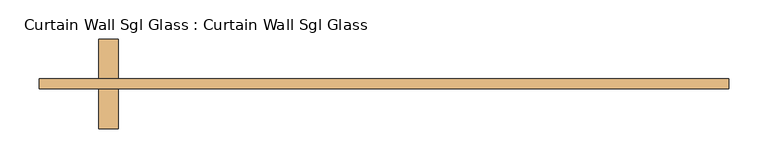
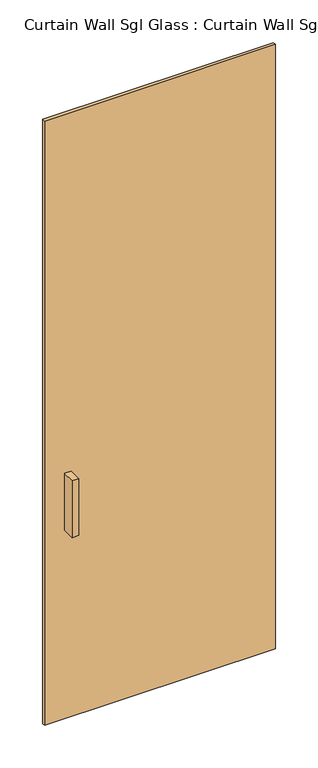
"""IFC4 building model written with IfcOpenShell, lengths in millimetres: door geometry, Curtain Wall Sgl Glass : Curtain Wall Sgl Glass."""

from ifc_helpers import new_model, si_unit, frame, origin, origin_with_axes, place, context, project, spatial, polyline, outline, extrude, source, transform, mapped, element, save


def curtain_wall_sgl_glass_curtain_wall_sgl_glass_0d6a1b13(model_context):
    return source(origin(), model_context, "Body", "SweptSolid", [
        extrude(outline(polyline([(-339.725, -12.7), (-365.125, -12.7), (-365.125, 38.1), (-339.725, 38.1), (-339.725, -12.7)])), frame((0.0, 0.0, 762.0), z_axis=(0.0, 0.0, 1.0), x_axis=(1.0, 0.0, 0.0)), (0.0, 0.0, 1.0), 228.6),
        extrude(outline(polyline([(-365.125, 101.6), (-339.725, 101.6), (-339.725, 50.8), (-365.125, 50.8), (-365.125, 101.6)])), frame((0.0, 0.0, 762.0), z_axis=(0.0, 0.0, 1.0), x_axis=(1.0, 0.0, 0.0)), (0.0, 0.0, 1.0), 228.6),
        extrude(outline(polyline([(441.325, 50.8), (441.325, 38.1), (-441.325, 38.1), (-441.325, 50.8), (441.325, 50.8)])), origin_with_axes(), (0.0, 0.0, 1.0), 2438.4),
    ])


if __name__ == "__main__":
    model = new_model("IFC4")
    model_context = context("Model", 3, world=origin())
    ifc_project = project(units=[si_unit("LENGTHUNIT", "METRE", prefix="MILLI")], contexts=[model_context])
    site = spatial("IfcSite", under=ifc_project)
    building = spatial("IfcBuilding", under=site)
    placement = place(None, origin())
    curtain_wall_sgl_glass_curtain_wall_sgl_glass_shape = curtain_wall_sgl_glass_curtain_wall_sgl_glass_0d6a1b13(model_context)
    element("IfcDoor", 1, ObjectType="Curtain Wall Sgl Glass : Curtain Wall Sgl Glass", at=placement, inside=building, context=model_context, shape_type="MappedRepresentation", body=[
        mapped(curtain_wall_sgl_glass_curtain_wall_sgl_glass_shape, transform((0.0, 0.0, 0.0), x_axis=(1.0, 0.0, 0.0), y_axis=(0.0, 1.0, 0.0), z_axis=(0.0, 0.0, 1.0))),
    ])
    save(model, "model.ifc")

# Revit data of these elements
# Type "Curtain Wall Sgl Glass : Curtain Wall Sgl Glass"
#   Type Mark = "8"
#   Assembly Code = "B2030100"
#   Thickness = 50.8 mm
#   Offset = 50.8 mm
#   Define Thermal Properties by = 0
#   Function = 1
#   Handle Material = Metal - Aluminum
#   Glazing Material = Glass
# Element 1 (IfcDoor, "Curtain Wall Sgl Glass : Curtain Wall Sgl Glass")
#   Materials on its faces: "Metal - Aluminum", "Glass"
# Materials
#   "Metal - Aluminum": class "Metal", colour RGB 247 247 247, transparency 0, Cost = 0
#   "Glass": class "Glass", colour RGB 154 182 205, transparency 0.5, Cost = 0
